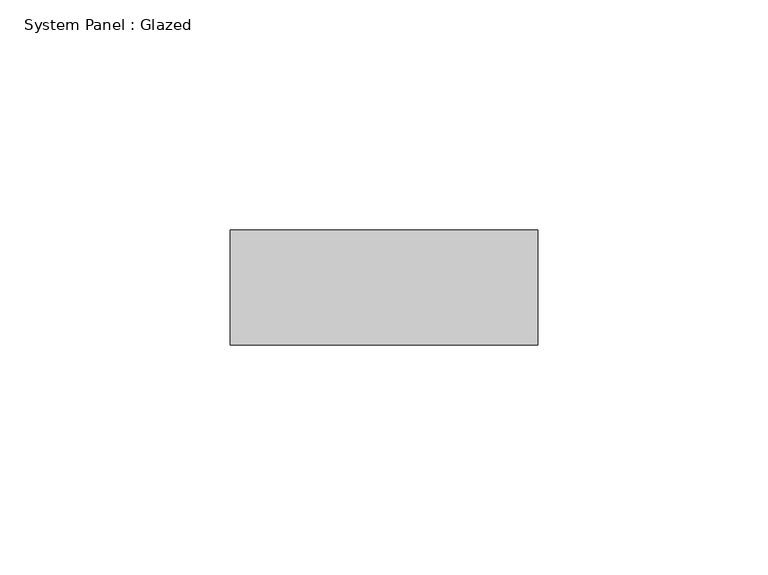
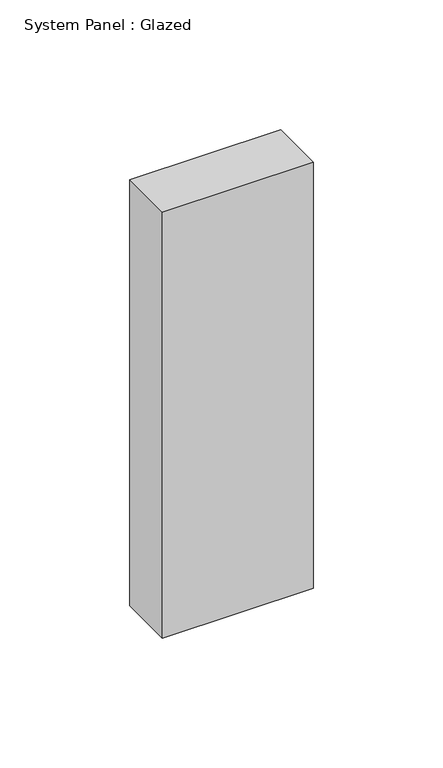
"""IFC4 building model written with IfcOpenShell, lengths in millimetres: plate geometry, System Panel : Glazed."""

from ifc_helpers import new_model, si_unit, origin, origin_with_axes, place, context, project, spatial, polyline, outline, extrude, source, transform, mapped, element, save


def system_panel_glazed_52e3984b(model_context):
    return source(origin(), model_context, "Body", "SweptSolid", [
        extrude(outline(polyline([(33.4301315, 24.5), (-33.4301315, 24.5), (-33.4301315, 49.5), (33.4301315, 49.5), (33.4301315, 24.5)])), origin_with_axes(), (0.0, 0.0, 1.0), 200.0),
    ])


if __name__ == "__main__":
    model = new_model("IFC4")
    model_context = context("Model", 3, world=origin())
    ifc_project = project(units=[si_unit("LENGTHUNIT", "METRE", prefix="MILLI")], contexts=[model_context])
    site = spatial("IfcSite", under=ifc_project)
    building = spatial("IfcBuilding", under=site)
    placement = place(None, origin())
    system_panel_glazed_shape = system_panel_glazed_52e3984b(model_context)
    element("IfcPlate", 1, ObjectType="System Panel : Glazed", at=placement, inside=building, context=model_context, shape_type="MappedRepresentation", body=[
        mapped(system_panel_glazed_shape, transform((0.0, 0.0, 0.0), x_axis=(1.0, 0.0, 0.0), y_axis=(0.0, 1.0, 0.0), z_axis=(0.0, 0.0, 1.0))),
    ])
    save(model, "model.ifc")

# Revit data of these elements
# Element 1 (IfcPlate, "System Panel : Glazed")
#   Materials on its faces: "Glass"
# Materials
#   "Glass": class "Glass", colour RGB 218 227 224, transparency 0.85, Description = "Soda Lime Glass", Cost = 0
